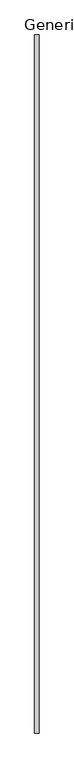
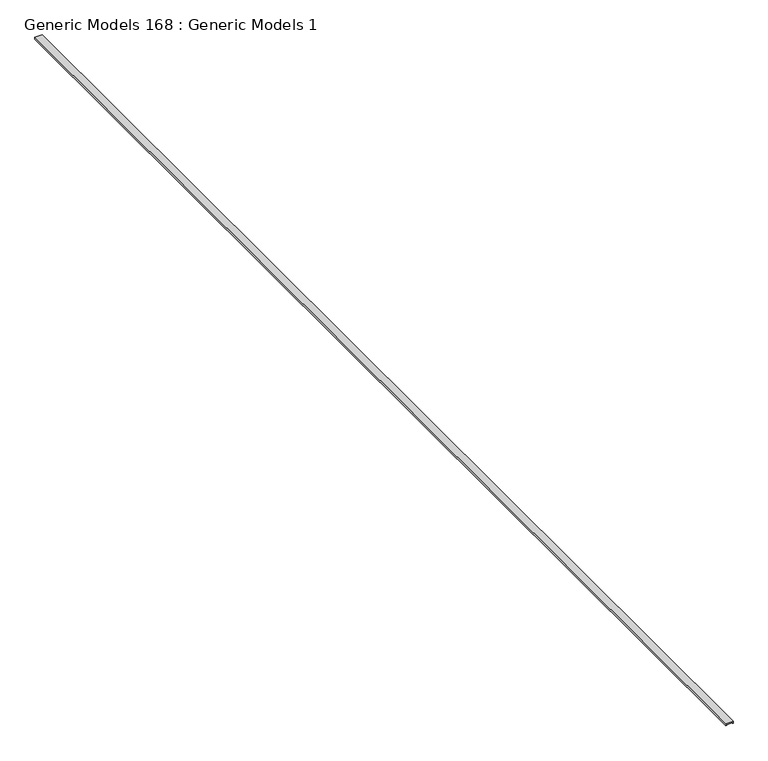
"""IFC4 building model written with IfcOpenShell, lengths in millimetres: proxy geometry, Generic Models 168 : Generic Models 1."""

import ifcopenshell
import ifcopenshell.guid

model = None  # the IFC model being written
_history = None  # IfcOwnerHistory: only IFC2X3 demands one
_inside = {}  # id of a spatial element -> (the spatial element, [elements in it])
_under = {}  # id of a project, library or spatial element -> (it, [spatial elements below it])
_declared = {}  # id of a project -> (the project, [libraries it declares])
_typed = {}  # id of a type object -> (the type object, [elements of that type])
_made_of = {}  # id of a material, layer set ... -> (it, [elements and type objects made of it])


def new_model(schema):
    """Start an empty IFC model of exactly this schema.

    Asked for "IFC4X3", IfcOpenShell would pick the latest addendum, in which some entities
    have other attributes; the version numbers below select the first issue.
    IFC2X3 requires an IfcOwnerHistory on every rooted entity: one is made here for all.
    """
    global model, _history
    if schema == "IFC4X3":
        model = ifcopenshell.file(schema_version=(4, 3, 0, 0))
    else:
        model = ifcopenshell.file(schema=schema)
    _inside.clear()
    _under.clear()
    _declared.clear()
    _typed.clear()
    _made_of.clear()
    _history = None
    if model.schema == "IFC2X3":
        org = make("IfcOrganization", Name="unknown")
        user = make(
            "IfcPersonAndOrganization",
            ThePerson=make("IfcPerson", FamilyName="unknown"),
            TheOrganization=org,
        )
        app = make(
            "IfcApplication",
            ApplicationDeveloper=org,
            Version="unknown",
            ApplicationFullName="unknown",
            ApplicationIdentifier="unknown",
        )
        _history = make(
            "IfcOwnerHistory",
            OwningUser=user,
            OwningApplication=app,
            ChangeAction="ADDED",
            CreationDate=0,
        )
    return model


def make(cls, **values):
    """One entity of the class cls with the attributes given. An attribute that is None is left unset."""
    return model.create_entity(
        cls, **{name: value for name, value in values.items() if value is not None}
    )


def rooted(cls, **values):
    """An entity with a GlobalId (a new one), such as an element, a storey or a relation."""
    return make(cls, GlobalId=ifcopenshell.guid.new(), OwnerHistory=_history, **values)


def si_unit(unit_type, name, prefix=None):
    """IfcSIUnit, for example si_unit("LENGTHUNIT", "METRE", prefix="MILLI")."""
    return make("IfcSIUnit", UnitType=unit_type, Prefix=prefix, Name=name)


def assignment(units):
    """IfcUnitAssignment: the units of a project."""
    return None if units is None else make("IfcUnitAssignment", Units=units)


def point(xyz):
    """IfcCartesianPoint."""
    return None if xyz is None else make("IfcCartesianPoint", Coordinates=xyz)


def direction(xyz):
    """IfcDirection."""
    return None if xyz is None else make("IfcDirection", DirectionRatios=xyz)


def frame(location, z_axis=None, x_axis=None):
    """IfcAxis2Placement3D, a coordinate frame: its origin and axes. An axis left out is left unset."""
    return make(
        "IfcAxis2Placement3D",
        Location=point(location),
        Axis=direction(z_axis),
        RefDirection=direction(x_axis),
    )


def origin():
    """The frame at (0, 0, 0) with its axes left unset."""
    return frame((0.0, 0.0, 0.0))


def place(relative_to, where):
    """IfcLocalPlacement: puts the frame where relative to a parent placement (None: the world)."""
    return make(
        "IfcLocalPlacement", PlacementRelTo=relative_to, RelativePlacement=where
    )


def context(
    kind, dimensions, precision=None, world=None, true_north=None, identifier=None
):
    """IfcGeometricRepresentationContext, for example the 3D "Model" context."""
    return make(
        "IfcGeometricRepresentationContext",
        ContextIdentifier=identifier,
        ContextType=kind,
        CoordinateSpaceDimension=dimensions,
        Precision=precision,
        WorldCoordinateSystem=world,
        TrueNorth=true_north,
    )


def project(units=None, contexts=None):
    """IfcProject with its units and contexts."""
    return rooted(
        "IfcProject",
        Name="project",
        RepresentationContexts=contexts,
        UnitsInContext=assignment(units),
    )


def spatial(cls, under=None, at=None, **own):
    """A site, building, storey or space (cls), placed at a placement, below another one or the project."""
    s = rooted(cls, ObjectPlacement=at, **own)
    if under is not None:
        _under.setdefault(under.id(), (under, []))[1].append(s)
    return s


def polyline(points):
    """IfcPolyline through the points."""
    return make("IfcPolyline", Points=[point(p) for p in points])


def outline(outer, holes=None, kind="AREA"):
    """IfcArbitraryClosedProfileDef: a profile drawn as a closed curve; with holes, ...WithVoids."""
    if holes is None:
        return make("IfcArbitraryClosedProfileDef", ProfileType=kind, OuterCurve=outer)
    return make(
        "IfcArbitraryProfileDefWithVoids",
        ProfileType=kind,
        OuterCurve=outer,
        InnerCurves=holes,
    )


def extrude(swept, where, along, depth):
    """IfcExtrudedAreaSolid: the profile swept, set in the frame where, extruded along a direction by depth."""
    return make(
        "IfcExtrudedAreaSolid",
        SweptArea=swept,
        Position=where,
        ExtrudedDirection=direction(along),
        Depth=depth,
    )


def shape(context_of_items, identifier, shape_type, items):
    """IfcShapeRepresentation: the items that make up one representation, for example the "Body"."""
    return make(
        "IfcShapeRepresentation",
        ContextOfItems=context_of_items,
        RepresentationIdentifier=identifier,
        RepresentationType=shape_type,
        Items=items,
    )


def source(mapping_origin, context_of_items, identifier, shape_type, items):
    """IfcRepresentationMap: a shape defined once, which mapped items show again and again."""
    return make(
        "IfcRepresentationMap",
        MappingOrigin=mapping_origin,
        MappedRepresentation=shape(context_of_items, identifier, shape_type, items),
    )


def transform(
    local_origin,
    x_axis=None,
    y_axis=None,
    z_axis=None,
    scale=None,
    scale2=None,
    scale3=None,
    uniform=True,
):
    """IfcCartesianTransformationOperator3D, or its non-uniform kind. x_axis, y_axis, z_axis: its Axis1, 2, 3."""
    if uniform:
        return make(
            "IfcCartesianTransformationOperator3D",
            Axis1=direction(x_axis),
            Axis2=direction(y_axis),
            LocalOrigin=point(local_origin),
            Scale=scale,
            Axis3=direction(z_axis),
        )
    return make(
        "IfcCartesianTransformationOperator3DnonUniform",
        Axis1=direction(x_axis),
        Axis2=direction(y_axis),
        LocalOrigin=point(local_origin),
        Scale=scale,
        Axis3=direction(z_axis),
        Scale2=scale2,
        Scale3=scale3,
    )


def mapped(mapping_source, mapping_target):
    """IfcMappedItem: shows the shape of a source again, moved by a transform."""
    return make(
        "IfcMappedItem", MappingSource=mapping_source, MappingTarget=mapping_target
    )


def made_of(thing, what):
    """Note that an element or type object is made of a material, layer set ...; save() writes the relation."""
    if what is not None:
        _made_of.setdefault(what.id(), (what, []))[1].append(thing)
    return thing


def element(
    cls,
    number,
    at=None,
    inside=None,
    cuts=None,
    type_object=None,
    material=None,
    context=None,
    identifier="Body",
    shape_type=None,
    held_by="IfcProductDefinitionShape",
    body=None,
    shapes=None,
    **own,
):
    """One element of the class cls, such as IfcWall. Its Tag is "e" and its number.

    at: its placement. inside: the storey or other place that contains it. cuts: it is an
    opening in that element (IfcRelVoidsElement). A single representation is given by context,
    identifier, shape_type and body (its items); several are given by shapes. held_by: the class
    of the entity that holds the representations. save() writes the other relations.
    """
    e = rooted(cls, Tag="e%d" % number, ObjectPlacement=at, **own)
    if body is not None:
        shapes = [shape(context, identifier, shape_type, body)]
    if shapes is not None:
        e.Representation = make(held_by, Representations=shapes)
    if inside is not None:
        _inside.setdefault(inside.id(), (inside, []))[1].append(e)
    if cuts is not None:
        rooted(
            "IfcRelVoidsElement", RelatingBuildingElement=cuts, RelatedOpeningElement=e
        )
    if type_object is not None:
        _typed.setdefault(type_object.id(), (type_object, []))[1].append(e)
    return made_of(e, material)


def aggregate(whole, parts):
    """IfcRelAggregates: a whole, such as a stair, and the parts it consists of."""
    return rooted("IfcRelAggregates", RelatingObject=whole, RelatedObjects=parts)


def save(model, path):
    """Write the relations noted so far, then the file.

    IfcRelAggregates (storeys below a building ...), IfcRelContainedInSpatialStructure (elements
    in a storey), IfcRelDefinesByType, IfcRelAssociatesMaterial and IfcRelDeclares: one each for
    every whole, place, type object, material and project.
    """
    for whole, parts in _under.values():
        aggregate(whole, parts)
    for where, things in _inside.values():
        rooted(
            "IfcRelContainedInSpatialStructure",
            RelatedElements=things,
            RelatingStructure=where,
        )
    for kind, things in _typed.values():
        rooted("IfcRelDefinesByType", RelatedObjects=things, RelatingType=kind)
    for what, things in _made_of.values():
        rooted("IfcRelAssociatesMaterial", RelatedObjects=things, RelatingMaterial=what)
    for by, libraries in _declared.values():
        rooted("IfcRelDeclares", RelatingContext=by, RelatedDefinitions=libraries)
    model.write(path)


def generic_models_168_generic_models_1_2062cc13(model_context):
    return source(origin(), model_context, "Body", "SweptSolid", [
        extrude(outline(polyline([(127853.384216, -8221.8361296), (127853.384216, -8288.5111296), (127834.334216, -8288.5111296), (127834.334216, -8280.5736296), (127840.684216, -8280.5736296), (127840.684216, -8229.7736296), (127834.334216, -8229.7736296), (127834.334216, -8221.8361296), (127853.384216, -8221.8361296)])), frame((0.0, -1999.2456111, 0.0), z_axis=(0.0, 1.0, 0.0), x_axis=(0.0, 0.0, 1.0)), (0.0, 0.0, 1.0), 10820.4),
    ])


if __name__ == "__main__":
    model = new_model("IFC4")
    model_context = context("Model", 3, world=origin())
    ifc_project = project(units=[si_unit("LENGTHUNIT", "METRE", prefix="MILLI")], contexts=[model_context])
    site = spatial("IfcSite", under=ifc_project)
    building = spatial("IfcBuilding", under=site)
    placement = place(None, origin())
    generic_models_168_generic_models_1_shape = generic_models_168_generic_models_1_2062cc13(model_context)
    element("IfcBuildingElementProxy", 1, Name="Generic Models 168 : Generic Models 1", ObjectType="Generic Models 168 : Generic Models 1", at=placement, inside=building, context=model_context, shape_type="MappedRepresentation", body=[
        mapped(generic_models_168_generic_models_1_shape, transform((0.0, 0.0, 0.0), x_axis=(1.0, 0.0, 0.0), y_axis=(0.0, 1.0, 0.0), z_axis=(0.0, 0.0, 1.0))),
    ])
    save(model, "model.ifc")

# Revit data of these elements
# Element 1 (IfcBuildingElementProxy, "Generic Models 168 : Generic Models 1")
#   Materials on its faces: "_2 5/8\" X 3/4\" WOOD TOP RAIL / HAND RAIL, EASE EDGES W/ .01 RADIUS"
# Materials
#   "_2 5/8\" X 3/4\" WOOD TOP RAIL / HAND RAIL, EASE EDGES W/ .01 RADIUS": class "Generic", colour RGB 177 130 114, transparency 0, Cost = 0
